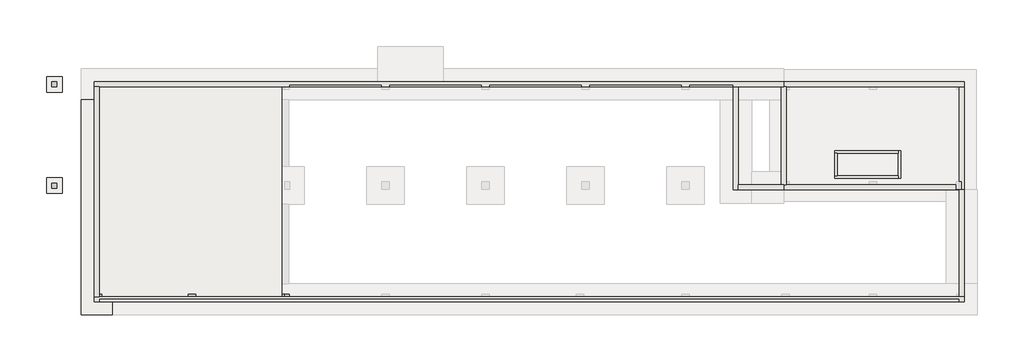
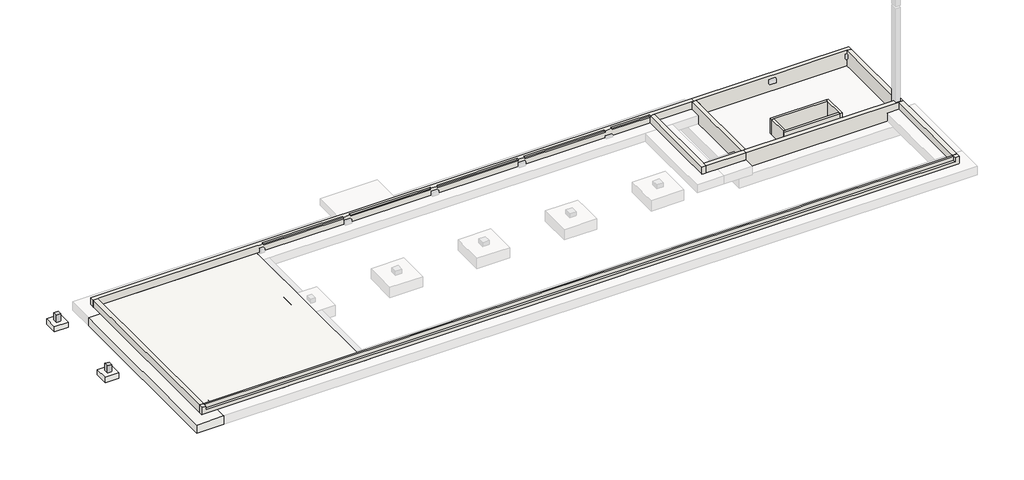
# Not in any storey, part 1 of 2: 14 walls, 5 columns, 3 slabs, 2 beams, 1 footing.
"""IFC4 building model written with IfcOpenShell, lengths in millimetres."""

import ifcopenshell
import ifcopenshell.guid

model = None  # the IFC model being written
_history = None  # IfcOwnerHistory: only IFC2X3 demands one
_inside = {}  # id of a spatial element -> (the spatial element, [elements in it])
_under = {}  # id of a project, library or spatial element -> (it, [spatial elements below it])
_declared = {}  # id of a project -> (the project, [libraries it declares])
_typed = {}  # id of a type object -> (the type object, [elements of that type])
_made_of = {}  # id of a material, layer set ... -> (it, [elements and type objects made of it])


def new_model(schema):
    """Start an empty IFC model of exactly this schema.

    Asked for "IFC4X3", IfcOpenShell would pick the latest addendum, in which some entities
    have other attributes; the version numbers below select the first issue.
    IFC2X3 requires an IfcOwnerHistory on every rooted entity: one is made here for all.
    """
    global model, _history
    if schema == "IFC4X3":
        model = ifcopenshell.file(schema_version=(4, 3, 0, 0))
    else:
        model = ifcopenshell.file(schema=schema)
    _inside.clear()
    _under.clear()
    _declared.clear()
    _typed.clear()
    _made_of.clear()
    _history = None
    if model.schema == "IFC2X3":
        org = make("IfcOrganization", Name="unknown")
        user = make(
            "IfcPersonAndOrganization",
            ThePerson=make("IfcPerson", FamilyName="unknown"),
            TheOrganization=org,
        )
        app = make(
            "IfcApplication",
            ApplicationDeveloper=org,
            Version="unknown",
            ApplicationFullName="unknown",
            ApplicationIdentifier="unknown",
        )
        _history = make(
            "IfcOwnerHistory",
            OwningUser=user,
            OwningApplication=app,
            ChangeAction="ADDED",
            CreationDate=0,
        )
    return model


def make(cls, **values):
    """One entity of the class cls with the attributes given. An attribute that is None is left unset."""
    return model.create_entity(
        cls, **{name: value for name, value in values.items() if value is not None}
    )


def rooted(cls, **values):
    """An entity with a GlobalId (a new one), such as an element, a storey or a relation."""
    return make(cls, GlobalId=ifcopenshell.guid.new(), OwnerHistory=_history, **values)


def si_unit(unit_type, name, prefix=None):
    """IfcSIUnit, for example si_unit("LENGTHUNIT", "METRE", prefix="MILLI")."""
    return make("IfcSIUnit", UnitType=unit_type, Prefix=prefix, Name=name)


def assignment(units):
    """IfcUnitAssignment: the units of a project."""
    return None if units is None else make("IfcUnitAssignment", Units=units)


def point(xyz):
    """IfcCartesianPoint."""
    return None if xyz is None else make("IfcCartesianPoint", Coordinates=xyz)


def direction(xyz):
    """IfcDirection."""
    return None if xyz is None else make("IfcDirection", DirectionRatios=xyz)


def frame(location, z_axis=None, x_axis=None):
    """IfcAxis2Placement3D, a coordinate frame: its origin and axes. An axis left out is left unset."""
    return make(
        "IfcAxis2Placement3D",
        Location=point(location),
        Axis=direction(z_axis),
        RefDirection=direction(x_axis),
    )


def origin():
    """The frame at (0, 0, 0) with its axes left unset."""
    return frame((0.0, 0.0, 0.0))


def place(relative_to, where):
    """IfcLocalPlacement: puts the frame where relative to a parent placement (None: the world)."""
    return make(
        "IfcLocalPlacement", PlacementRelTo=relative_to, RelativePlacement=where
    )


def context(
    kind, dimensions, precision=None, world=None, true_north=None, identifier=None
):
    """IfcGeometricRepresentationContext, for example the 3D "Model" context."""
    return make(
        "IfcGeometricRepresentationContext",
        ContextIdentifier=identifier,
        ContextType=kind,
        CoordinateSpaceDimension=dimensions,
        Precision=precision,
        WorldCoordinateSystem=world,
        TrueNorth=true_north,
    )


def project(units=None, contexts=None):
    """IfcProject with its units and contexts."""
    return rooted(
        "IfcProject",
        Name="project",
        RepresentationContexts=contexts,
        UnitsInContext=assignment(units),
    )


def spatial(cls, under=None, at=None, **own):
    """A site, building, storey or space (cls), placed at a placement, below another one or the project."""
    s = rooted(cls, ObjectPlacement=at, **own)
    if under is not None:
        _under.setdefault(under.id(), (under, []))[1].append(s)
    return s


def polyline(points):
    """IfcPolyline through the points."""
    return make("IfcPolyline", Points=[point(p) for p in points])


def outline(outer, holes=None, kind="AREA"):
    """IfcArbitraryClosedProfileDef: a profile drawn as a closed curve; with holes, ...WithVoids."""
    if holes is None:
        return make("IfcArbitraryClosedProfileDef", ProfileType=kind, OuterCurve=outer)
    return make(
        "IfcArbitraryProfileDefWithVoids",
        ProfileType=kind,
        OuterCurve=outer,
        InnerCurves=holes,
    )


def extrude(swept, where, along, depth):
    """IfcExtrudedAreaSolid: the profile swept, set in the frame where, extruded along a direction by depth."""
    return make(
        "IfcExtrudedAreaSolid",
        SweptArea=swept,
        Position=where,
        ExtrudedDirection=direction(along),
        Depth=depth,
    )


def faces_of(points, faces, orient=None, outer=None):
    """IfcFace entities. A face is a list of loops; a loop is a list of indices into points, from 0.

    orient and outer hold one flag for each loop. By default every Orientation is true, the
    first loop of a face is its IfcFaceOuterBound and the others are IfcFaceBound.
    """
    made = []
    for i, loops in enumerate(faces):
        bounds = []
        for j, loop in enumerate(loops):
            is_outer = j == 0 if outer is None else outer[i][j]
            bounds.append(
                make(
                    "IfcFaceOuterBound" if is_outer else "IfcFaceBound",
                    Bound=make("IfcPolyLoop", Polygon=[points[k] for k in loop]),
                    Orientation=True if orient is None else orient[i][j],
                )
            )
        made.append(make("IfcFace", Bounds=bounds))
    return made


def faceted_brep(points, faces, orient=None, outer=None, voids=None):
    """IfcFacetedBrep: a solid bounded by flat faces; with voids (closed shells), ...WithVoids."""
    shared = [point(p) for p in points]
    hull = make("IfcClosedShell", CfsFaces=faces_of(shared, faces, orient, outer))
    if voids is None:
        return make("IfcFacetedBrep", Outer=hull)
    return make(
        "IfcFacetedBrepWithVoids",
        Outer=hull,
        Voids=[
            make(cls, CfsFaces=faces_of(shared, fs, o, b)) for cls, fs, o, b in voids
        ],
    )


def shape(context_of_items, identifier, shape_type, items):
    """IfcShapeRepresentation: the items that make up one representation, for example the "Body"."""
    return make(
        "IfcShapeRepresentation",
        ContextOfItems=context_of_items,
        RepresentationIdentifier=identifier,
        RepresentationType=shape_type,
        Items=items,
    )


def source(mapping_origin, context_of_items, identifier, shape_type, items):
    """IfcRepresentationMap: a shape defined once, which mapped items show again and again."""
    return make(
        "IfcRepresentationMap",
        MappingOrigin=mapping_origin,
        MappedRepresentation=shape(context_of_items, identifier, shape_type, items),
    )


def transform(
    local_origin,
    x_axis=None,
    y_axis=None,
    z_axis=None,
    scale=None,
    scale2=None,
    scale3=None,
    uniform=True,
):
    """IfcCartesianTransformationOperator3D, or its non-uniform kind. x_axis, y_axis, z_axis: its Axis1, 2, 3."""
    if uniform:
        return make(
            "IfcCartesianTransformationOperator3D",
            Axis1=direction(x_axis),
            Axis2=direction(y_axis),
            LocalOrigin=point(local_origin),
            Scale=scale,
            Axis3=direction(z_axis),
        )
    return make(
        "IfcCartesianTransformationOperator3DnonUniform",
        Axis1=direction(x_axis),
        Axis2=direction(y_axis),
        LocalOrigin=point(local_origin),
        Scale=scale,
        Axis3=direction(z_axis),
        Scale2=scale2,
        Scale3=scale3,
    )


def mapped(mapping_source, mapping_target):
    """IfcMappedItem: shows the shape of a source again, moved by a transform."""
    return make(
        "IfcMappedItem", MappingSource=mapping_source, MappingTarget=mapping_target
    )


def made_of(thing, what):
    """Note that an element or type object is made of a material, layer set ...; save() writes the relation."""
    if what is not None:
        _made_of.setdefault(what.id(), (what, []))[1].append(thing)
    return thing


def element(
    cls,
    number,
    at=None,
    inside=None,
    cuts=None,
    type_object=None,
    material=None,
    context=None,
    identifier="Body",
    shape_type=None,
    held_by="IfcProductDefinitionShape",
    body=None,
    shapes=None,
    **own,
):
    """One element of the class cls, such as IfcWall. Its Tag is "e" and its number.

    at: its placement. inside: the storey or other place that contains it. cuts: it is an
    opening in that element (IfcRelVoidsElement). A single representation is given by context,
    identifier, shape_type and body (its items); several are given by shapes. held_by: the class
    of the entity that holds the representations. save() writes the other relations.
    """
    e = rooted(cls, Tag="e%d" % number, ObjectPlacement=at, **own)
    if body is not None:
        shapes = [shape(context, identifier, shape_type, body)]
    if shapes is not None:
        e.Representation = make(held_by, Representations=shapes)
    if inside is not None:
        _inside.setdefault(inside.id(), (inside, []))[1].append(e)
    if cuts is not None:
        rooted(
            "IfcRelVoidsElement", RelatingBuildingElement=cuts, RelatedOpeningElement=e
        )
    if type_object is not None:
        _typed.setdefault(type_object.id(), (type_object, []))[1].append(e)
    return made_of(e, material)


def aggregate(whole, parts):
    """IfcRelAggregates: a whole, such as a stair, and the parts it consists of."""
    return rooted("IfcRelAggregates", RelatingObject=whole, RelatedObjects=parts)


def save(model, path):
    """Write the relations noted so far, then the file.

    IfcRelAggregates (storeys below a building ...), IfcRelContainedInSpatialStructure (elements
    in a storey), IfcRelDefinesByType, IfcRelAssociatesMaterial and IfcRelDeclares: one each for
    every whole, place, type object, material and project.
    """
    for whole, parts in _under.values():
        aggregate(whole, parts)
    for where, things in _inside.values():
        rooted(
            "IfcRelContainedInSpatialStructure",
            RelatedElements=things,
            RelatingStructure=where,
        )
    for kind, things in _typed.values():
        rooted("IfcRelDefinesByType", RelatedObjects=things, RelatingType=kind)
    for what, things in _made_of.values():
        rooted("IfcRelAssociatesMaterial", RelatedObjects=things, RelatingMaterial=what)
    for by, libraries in _declared.values():
        rooted("IfcRelDeclares", RelatingContext=by, RelatedDefinitions=libraries)
    model.write(path)


def foundation_rectangular_non_pile_17b72d6a(model_context):
    return source(origin(), model_context, "Body", "SweptSolid", [
        extrude(outline(polyline([(625.0, 625.0), (625.0, -625.0), (-625.0, -625.0), (-625.0, 625.0), (625.0, 625.0)])), frame((0.0, 0.0, -500.0), z_axis=(0.0, 0.0, 1.0), x_axis=(1.0, 0.0, 0.0)), (0.0, 0.0, 1.0), 500.0),
    ])


model = new_model("IFC4")

# Units and contexts
model_context = context("Model", 3, world=origin())
ifc_project = project(units=[si_unit("LENGTHUNIT", "METRE", prefix="MILLI")], contexts=[model_context])

# Site, building
site = spatial("IfcSite", under=ifc_project)
building = spatial("IfcBuilding", under=site)

# Beams
placement = place(None, origin())
element("IfcBeam", 1, ObjectType="RC Beam_Rectangular : H_SB_AR_S16_FG_B500xH700_FB1", at=placement, inside=building, context=model_context, shape_type="SweptSolid", body=[
    extrude(outline(polyline([(3500.0, 9199.5208589), (4000.0, 9199.5208589), (4000.0, 1649.5208589), (3500.0, 1649.5208589), (3500.0, 9199.5208589)])), frame((0.0, 0.0, -1250.0381366), z_axis=(0.0, 0.0, 1.0), x_axis=(1.0, 0.0, 0.0)), (0.0, 0.0, 1.0), 550.0),
])
element("IfcBeam", 2, ObjectType="RC Beam_Rectangular : H_SB_AR_S16_FG_B500xH700_FG1", at=placement, inside=building, context=model_context, shape_type="SweptSolid", body=[
    extrude(outline(polyline([(7750.0, 1649.5208589), (7250.0, 1649.5208589), (7250.0, 7999.5208589), (7750.0, 7999.5208589), (7750.0, 1649.5208589)])), frame((0.0, 0.0, -1250.0381366), z_axis=(0.0, 0.0, 1.0), x_axis=(1.0, 0.0, 0.0)), (0.0, 0.0, 1.0), 550.0),
])

# Columns
element("IfcColumn", 3, ObjectType="RC_Column_Rectangular : H_SC_AR_S15_UG_W600xL600_C2", at=placement, inside=building, context=model_context, shape_type="Brep", body=[
    faceted_brep([(15300.0, 799.5208589, -850.0381366), (15300.0, 199.5208589, -850.0381366), (14700.0, 199.5208589, -850.0381366), (14700.0, 799.5208589, -850.0381366), (15300.0, 799.5208589, -150.0381366), (15300.0, 599.5208589, -150.0381366), (15300.0, 599.5208589, -550.0381366), (15300.0, 199.5208589, -550.0381366), (14700.0, 199.5208589, -550.0381366), (14700.0, 599.5208589, -550.0381366), (14700.0, 799.5208589, -550.0381366), (14950.0, 799.5208589, -550.0381366), (14950.0, 799.5208589, -150.0381366), (14950.0, 599.5208589, -150.0381366), (14950.0, 599.5208589, -550.0381366)], [[[0, 1, 2, 3]], [[1, 0, 4, 5, 6, 7]], [[2, 1, 7, 8]], [[3, 2, 8, 9, 10]], [[0, 3, 10, 11, 12, 4]], [[5, 4, 12, 13]], [[6, 5, 13, 14]], [[7, 6, 14, 11, 10, 9, 8]], [[11, 14, 13, 12]]]),
])
element("IfcColumn", 4, ObjectType="RC_Column_Rectangular : H_SC_AR_S15_UG_W600xL600_C2", at=placement, inside=building, context=model_context, shape_type="Brep", body=[
    faceted_brep([(7800.0, 799.5208589, -850.0381366), (7800.0, 199.5208589, -850.0381366), (7200.0, 199.5208589, -850.0381366), (7200.0, 799.5208589, -850.0381366), (7800.0, 599.5208589, -150.0381366), (7800.0, 599.5208589, -550.0381366), (7800.0, 799.5208589, -550.0381366), (7800.0, 799.5208589, -150.0381366), (7800.0, 199.5208589, -550.0381366), (7200.0, 199.5208589, -550.0381366), (7200.0, 599.5208589, -550.0381366), (7200.0, 599.5208589, -150.0381366), (7200.0, 799.5208589, -150.0381366), (7200.0, 799.5208589, -550.0381366), (7200.0, 599.5208589, -700.0381366), (7800.0, 599.5208589, -700.0381366), (7800.0, 799.5208589, -700.0381366), (7200.0, 799.5208589, -700.0381366)], [[[0, 1, 2, 3]], [[4, 5, 6, 7]], [[2, 1, 8, 9]], [[10, 11, 12, 13]], [[12, 7, 6, 13]], [[7, 12, 11, 4]], [[10, 5, 4, 11]], [[5, 10, 9, 8]], [[14, 15, 16, 17]], [[5, 10, 13, 6]], [[10, 5, 15, 14]], [[1, 0, 16, 15, 5, 8]], [[3, 2, 9, 10, 14, 17]], [[0, 3, 17, 16]]]),
])
element("IfcColumn", 5, ObjectType="RC_Column_Rectangular : H_SC_AR_S15_UG_W600xL600_C2", at=placement, inside=building, context=model_context, shape_type="Brep", body=[
    faceted_brep([(300.0, 799.5208589, -850.0381366), (300.0, 199.5208589, -850.0381366), (-300.0, 199.5208589, -850.0381366), (-300.0, 799.5208589, -850.0381366), (300.0, 599.5208589, -150.0381366), (300.0, 599.5208589, -550.0381366), (300.0, 799.5208589, -550.0381366), (300.0, 799.5208589, -150.0381366), (300.0, 199.5208589, -550.0381366), (-300.0, 199.5208589, -550.0381366), (-300.0, 599.5208589, -550.0381366), (-300.0, 799.5208589, -550.0381366), (100.0, 799.5208589, -550.0381366), (100.0, 799.5208589, -150.0381366), (100.0, 599.5208589, -150.0381366), (100.0, 599.5208589, -550.0381366), (100.0, 799.5208589, -700.0381366), (100.0, 599.5208589, -700.0381366), (300.0, 599.5208589, -700.0381366), (300.0, 799.5208589, -700.0381366), (100.0, 599.5208589, -550.0381366)], [[[0, 1, 2, 3]], [[4, 5, 6, 7]], [[2, 1, 8, 9]], [[3, 2, 9, 10, 11]], [[12, 13, 7, 6]], [[4, 7, 13, 14]], [[5, 4, 14, 15]], [[8, 5, 15, 12, 11, 10, 9]], [[12, 15, 14, 13]], [[16, 17, 18, 19]], [[5, 20, 12, 6]], [[17, 20, 5, 18]], [[20, 17, 16, 12]], [[1, 0, 19, 18, 5, 8]], [[0, 3, 11, 12, 16, 19]]]),
])
element("IfcColumn", 6, ObjectType="RC_Column_Rectangular : H_SC_AR_S15_UG_W400xL400_C3", at=placement, inside=building, context=model_context, shape_type="SweptSolid", body=[
    extrude(outline(polyline([(-3300.0, 9699.5208589), (-3300.0, 9299.5208589), (-3700.0, 9299.5208589), (-3700.0, 9699.5208589), (-3300.0, 9699.5208589)])), frame((0.0, 0.0, -850.0381366), z_axis=(0.0, 0.0, 1.0), x_axis=(1.0, 0.0, 0.0)), (0.0, 0.0, 1.0), 700.0),
])
element("IfcColumn", 7, ObjectType="RC_Column_Rectangular : H_SC_AR_S15_UG_W400xL400_C3", at=placement, inside=building, context=model_context, shape_type="Brep", body=[
    faceted_brep([(-3300.0, 17799.5208589, -850.0381366), (-3300.0, 17399.5208589, -850.0381366), (-3700.0, 17399.5208589, -850.0381366), (-3700.0, 17799.5208589, -850.0381366), (-3300.0, 17799.5208589, -150.0381366), (-3300.0, 17399.5208589, -150.0381366), (-3300.0, 17399.5208589, -550.0381366), (-3300.0, 17799.5208589, -550.0381366), (-3700.0, 17399.5208589, -150.0381366), (-3700.0, 17799.5208589, -150.0381366)], [[[0, 1, 2, 3]], [[4, 5, 6, 1, 0, 7]], [[5, 8, 2, 1, 6]], [[8, 9, 3, 2]], [[9, 4, 7, 0, 3]], [[4, 9, 8, 5]]]),
])

# Footing
element("IfcFooting", 8, ObjectType="H_SF_AR_B01_Wall FDN_T800", at=placement, inside=building, context=model_context, shape_type="Brep", body=[
    faceted_brep([(-1350.0, -850.4791411, -550.0381366), (1150.0, -850.4791411, -550.0381366), (1150.0, 1649.5208589, -550.0381366), (1150.0, 16349.5208589, -550.0381366), (-1350.0, 16349.5208589, -550.0381366), (-1350.0, -850.4791411, -1350.0381366), (-1350.0, 16349.5208589, -1350.0381366), (1150.0, -850.4791411, -1350.0381366), (1150.0, 16349.5208589, -1350.0381366), (1150.0, 9799.5208589, -1350.0381366), (1150.0, 9199.5208589, -1350.0381366), (1150.0, 1649.5208589, -1350.0381366)], [[[0, 1, 2, 3, 4]], [[5, 0, 4, 6]], [[7, 5, 6, 8, 9, 10, 11]], [[1, 7, 11, 10, 9, 8, 3, 2]], [[1, 0, 5, 7]], [[4, 3, 8, 6]]]),
])

# Slabs
element("IfcSlab", 9, ObjectType="H_FL_AR_S17_RC Slab T150_B1S1", at=placement, inside=building, context=model_context, shape_type="Brep", body=[
    faceted_brep([(14700.0, 17399.5208589, -700.0381366), (14700.0, 599.5208589, -700.0381366), (7800.0, 599.5208589, -700.0381366), (7200.0, 599.5208589, -700.0381366), (300.0, 599.5208589, -700.0381366), (100.0, 599.5208589, -700.0381366), (100.0, 799.5208589, -700.0381366), (100.0, 17199.5208589, -700.0381366), (100.0, 17399.5208589, -700.0381366), (300.0, 17399.5208589, -700.0381366), (7200.0, 17399.5208589, -700.0381366), (7800.0, 17399.5208589, -700.0381366), (14700.0, 17399.5208589, -550.0381366), (7800.0, 17399.5208589, -550.0381366), (7200.0, 17399.5208589, -550.0381366), (300.0, 17399.5208589, -550.0381366), (100.0, 17399.5208589, -550.0381366), (100.0, 17199.5208589, -550.0381366), (100.0, 799.5208589, -550.0381366), (100.0, 599.5208589, -550.0381366), (300.0, 599.5208589, -550.0381366), (7200.0, 599.5208589, -550.0381366), (7800.0, 599.5208589, -550.0381366), (14700.0, 599.5208589, -550.0381366), (14700.0, 799.5208589, -550.0381366), (14700.0, 17199.5208589, -550.0381366)], [[[0, 1, 2, 3, 4, 5, 6, 7, 8, 9, 10, 11]], [[12, 13, 14, 15, 16, 17, 18, 19, 20, 21, 22, 23, 24, 25]], [[1, 0, 12, 25, 24, 23]], [[5, 4, 3, 2, 1, 23, 22, 21, 20, 19]], [[8, 7, 6, 5, 19, 18, 17, 16]], [[0, 11, 10, 9, 8, 16, 15, 14, 13, 12]]]),
])
element("IfcSlab", 10, ObjectType="Foundation Rectangular (Non-Pile) : H_SF_AR_S18_W1250xL1250xT500_Bitumen_F2", at=placement, inside=building, context=model_context, shape_type="SweptSolid", body=[
    extrude(outline(polyline([(-2875.0, 18224.5208589), (-2875.0, 16974.5208589), (-4125.0, 16974.5208589), (-4125.0, 18224.5208589), (-2875.0, 18224.5208589)])), frame((0.0, 0.0, -1350.0381366), z_axis=(0.0, 0.0, 1.0), x_axis=(1.0, 0.0, 0.0)), (0.0, 0.0, 1.0), 500.0),
])
foundation_rectangular_non_pile_shape = foundation_rectangular_non_pile_17b72d6a(model_context)
element("IfcSlab", 11, ObjectType="Foundation Rectangular (Non-Pile) : H_SF_AR_S18_W1250xL1250xT500_Bitumen_F2", at=placement, inside=building, context=model_context, shape_type="MappedRepresentation", body=[
    mapped(foundation_rectangular_non_pile_shape, transform((-3500.0, 9499.5208589, -850.0381366), x_axis=(1.0, 0.0, 0.0), y_axis=(0.0, 1.0, 0.0), z_axis=(0.0, 0.0, 1.0))),
])

# Walls
element("IfcWall", 12, ObjectType="H_WA_AR_B02_Ext Wall_RC T400_UG_Bitumen 2", at=placement, inside=building, context=model_context, shape_type="Brep", body=[
    faceted_brep([(-300.0, 17399.5208589, -550.0381366), (100.0, 17399.5208589, -550.0381366), (300.0, 17399.5208589, -550.0381366), (7200.0, 17399.5208589, -550.0381366), (7800.0, 17399.5208589, -550.0381366), (14700.0, 17399.5208589, -550.0381366), (14950.0, 17399.5208589, -550.0381366), (15300.0, 17399.5208589, -550.0381366), (22700.0, 17399.5208589, -550.0381366), (23300.0, 17399.5208589, -550.0381366), (30700.0, 17399.5208589, -550.0381366), (31300.0, 17399.5208589, -550.0381366), (38700.0, 17399.5208589, -550.0381366), (39300.0, 17399.5208589, -550.0381366), (46700.0, 17399.5208589, -550.0381366), (47300.0, 17399.5208589, -550.0381366), (50825.0, 17399.5208589, -550.0381366), (51225.0, 17399.5208589, -550.0381366), (54650.0, 17399.5208589, -550.0381366), (54850.0, 17399.5208589, -550.0381366), (54850.0, 17399.5208589, 149.9618634), (54650.0, 17399.5208589, 149.9618634), (51225.0, 17399.5208589, 149.9618634), (50825.0, 17399.5208589, 149.9618634), (50825.0, 17399.5208589, -0.0381366), (47300.0, 17399.5208589, -0.0381366), (47300.0, 17399.5208589, 149.9618634), (46700.0, 17399.5208589, 149.9618634), (46700.0, 17399.5208589, -0.0381366), (39300.0, 17399.5208589, -0.0381366), (39300.0, 17399.5208589, 149.9618634), (38700.0, 17399.5208589, 149.9618634), (38700.0, 17399.5208589, -0.0381366), (31300.0, 17399.5208589, -0.0381366), (31300.0, 17399.5208589, 149.9618634), (30700.0, 17399.5208589, 149.9618634), (30700.0, 17399.5208589, -0.0381366), (23300.0, 17399.5208589, -0.0381366), (23300.0, 17399.5208589, 149.9618634), (22700.0, 17399.5208589, 149.9618634), (22700.0, 17399.5208589, -0.0381366), (15300.0, 17399.5208589, -0.0381366), (15300.0, 17399.5208589, 149.9618634), (14950.0, 17399.5208589, 149.9618634), (14700.0, 17399.5208589, 149.9618634), (7800.0, 17399.5208589, 149.9618634), (7200.0, 17399.5208589, 149.9618634), (300.0, 17399.5208589, 149.9618634), (100.0, 17399.5208589, 149.9618634), (-300.0, 17399.5208589, 149.9618634), (-300.0, 17399.5208589, -20.0381366), (54850.0, 17799.5208589, -550.0381366), (54650.0, 17799.5208589, -550.0381366), (47300.0, 17799.5208589, -550.0381366), (46700.0, 17799.5208589, -550.0381366), (39300.0, 17799.5208589, -550.0381366), (38700.0, 17799.5208589, -550.0381366), (31300.0, 17799.5208589, -550.0381366), (30700.0, 17799.5208589, -550.0381366), (23300.0, 17799.5208589, -550.0381366), (22700.0, 17799.5208589, -550.0381366), (15300.0, 17799.5208589, -550.0381366), (14700.0, 17799.5208589, -550.0381366), (7800.0, 17799.5208589, -550.0381366), (7200.0, 17799.5208589, -550.0381366), (300.0, 17799.5208589, -550.0381366), (-300.0, 17799.5208589, -550.0381366), (-300.0, 17799.5208589, -20.0381366), (-300.0, 17799.5208589, 149.9618634), (18450.0, 17799.5208589, 149.9618634), (19550.0, 17799.5208589, 149.9618634), (24050.0, 17799.5208589, 149.9618634), (26150.0, 17799.5208589, 149.9618634), (54850.0, 17799.5208589, 149.9618634), (-300.0, 17549.5208589, 149.9618634), (15300.0, 17549.5208589, 149.9618634), (22700.0, 17549.5208589, 149.9618634), (23300.0, 17549.5208589, 149.9618634), (30700.0, 17549.5208589, 149.9618634), (31300.0, 17549.5208589, 149.9618634), (38700.0, 17549.5208589, 149.9618634), (39300.0, 17549.5208589, 149.9618634), (46700.0, 17549.5208589, 149.9618634), (47300.0, 17549.5208589, 149.9618634), (50825.0, 17549.5208589, 149.9618634), (22700.0, 17549.5208589, -0.0381366), (15300.0, 17549.5208589, -0.0381366), (30700.0, 17549.5208589, -0.0381366), (23300.0, 17549.5208589, -0.0381366), (38700.0, 17549.5208589, -0.0381366), (31300.0, 17549.5208589, -0.0381366), (46700.0, 17549.5208589, -0.0381366), (39300.0, 17549.5208589, -0.0381366), (50825.0, 17549.5208589, -0.0381366), (47300.0, 17549.5208589, -0.0381366)], [[[0, 1, 2, 3, 4, 5, 6, 7, 8, 9, 10, 11, 12, 13, 14, 15, 16, 17, 18, 19, 20, 21, 22, 23, 24, 25, 26, 27, 28, 29, 30, 31, 32, 33, 34, 35, 36, 37, 38, 39, 40, 41, 42, 43, 44, 45, 46, 47, 48, 49, 50]], [[51, 52, 53, 54, 55, 56, 57, 58, 59, 60, 61, 62, 63, 64, 65, 66, 67, 68, 69, 70, 71, 72, 73]], [[19, 18, 17, 16, 15, 14, 13, 12, 11, 10, 9, 8, 7, 6, 5, 4, 3, 2, 1, 0, 66, 65, 64, 63, 62, 61, 60, 59, 58, 57, 56, 55, 54, 53, 52, 51]], [[20, 19, 51, 73]], [[73, 72, 71, 70, 69, 68, 74, 49, 48, 47, 46, 45, 44, 43, 42, 75, 76, 39, 38, 77, 78, 35, 34, 79, 80, 31, 30, 81, 82, 27, 26, 83, 84, 23, 22, 21, 20]], [[49, 74, 68, 67, 66, 0, 50]], [[85, 86, 41, 40]], [[87, 88, 37, 36]], [[89, 90, 33, 32]], [[91, 92, 29, 28]], [[93, 94, 25, 24]], [[86, 75, 42, 41]], [[86, 85, 76, 75]], [[76, 85, 40, 39]], [[88, 77, 38, 37]], [[88, 87, 78, 77]], [[78, 87, 36, 35]], [[90, 79, 34, 33]], [[90, 89, 80, 79]], [[80, 89, 32, 31]], [[92, 81, 30, 29]], [[92, 91, 82, 81]], [[82, 91, 28, 27]], [[94, 83, 26, 25]], [[94, 93, 84, 83]], [[84, 93, 24, 23]]]),
])
element("IfcWall", 13, ObjectType="H_WA_AR_B02_Ext Wall_RC T400_UG_Bitumen 2", at=placement, inside=building, context=model_context, shape_type="Brep", body=[
    faceted_brep([(69300.0, 599.5208589, -550.0381366), (68900.0, 599.5208589, -550.0381366), (68700.0, 599.5208589, -550.0381366), (62300.0, 599.5208589, -550.0381366), (61700.0, 599.5208589, -550.0381366), (55300.0, 599.5208589, -550.0381366), (54700.0, 599.5208589, -550.0381366), (47300.0, 599.5208589, -550.0381366), (46700.0, 599.5208589, -550.0381366), (39240.1112654, 599.5208589, -550.0381366), (38850.0, 599.5208589, -550.0381366), (38250.0, 599.5208589, -550.0381366), (31300.0, 599.5208589, -550.0381366), (30700.0, 599.5208589, -550.0381366), (23300.0, 599.5208589, -550.0381366), (22700.0, 599.5208589, -550.0381366), (15300.0, 599.5208589, -550.0381366), (14950.0, 599.5208589, -550.0381366), (14700.0, 599.5208589, -550.0381366), (7800.0, 599.5208589, -550.0381366), (7200.0, 599.5208589, -550.0381366), (300.0, 599.5208589, -550.0381366), (100.0, 599.5208589, -550.0381366), (-300.0, 599.5208589, -550.0381366), (-300.0, 599.5208589, 149.9618634), (100.0, 599.5208589, 149.9618634), (300.0, 599.5208589, 149.9618634), (7200.0, 599.5208589, 149.9618634), (7800.0, 599.5208589, 149.9618634), (14700.0, 599.5208589, 149.9618634), (14950.0, 599.5208589, 149.9618634), (15300.0, 599.5208589, 149.9618634), (22700.0, 599.5208589, 149.9618634), (23300.0, 599.5208589, 149.9618634), (30700.0, 599.5208589, 149.9618634), (31300.0, 599.5208589, 149.9618634), (38700.0, 599.5208589, 149.9618634), (39300.0, 599.5208589, 149.9618634), (46700.0, 599.5208589, 149.9618634), (47300.0, 599.5208589, 149.9618634), (54700.0, 599.5208589, 149.9618634), (55300.0, 599.5208589, 149.9618634), (61700.0, 599.5208589, 149.9618634), (62300.0, 599.5208589, 149.9618634), (68700.0, 599.5208589, 149.9618634), (68900.0, 599.5208589, 149.9618634), (69300.0, 599.5208589, 149.9618634), (-300.0, 199.5208589, -550.0381366), (300.0, 199.5208589, -550.0381366), (7200.0, 199.5208589, -550.0381366), (7800.0, 199.5208589, -550.0381366), (14700.0, 199.5208589, -550.0381366), (15300.0, 199.5208589, -550.0381366), (22700.0, 199.5208589, -550.0381366), (23300.0, 199.5208589, -550.0381366), (30700.0, 199.5208589, -550.0381366), (31300.0, 199.5208589, -550.0381366), (38250.0, 199.5208589, -550.0381366), (38850.0, 199.5208589, -550.0381366), (46700.0, 199.5208589, -550.0381366), (47300.0, 199.5208589, -550.0381366), (54700.0, 199.5208589, -550.0381366), (55300.0, 199.5208589, -550.0381366), (61700.0, 199.5208589, -550.0381366), (62300.0, 199.5208589, -550.0381366), (68700.0, 199.5208589, -550.0381366), (69300.0, 199.5208589, -550.0381366), (69300.0, 199.5208589, 149.9618634), (68900.0, 199.5208589, 149.9618634), (68900.0, 199.5208589, -231.142699), (100.0, 199.5208589, -231.142699), (100.0, 199.5208589, 149.9618634), (-50.0, 199.5208589, 149.9618634), (-300.0, 199.5208589, 149.9618634), (100.0, 449.5208589, 149.9618634), (300.0, 449.5208589, 149.9618634), (7200.0, 449.5208589, 149.9618634), (7800.0, 449.5208589, 149.9618634), (14700.0, 449.5208589, 149.9618634), (15300.0, 449.5208589, 149.9618634), (22700.0, 449.5208589, 149.9618634), (23300.0, 449.5208589, 149.9618634), (30700.0, 449.5208589, 149.9618634), (31300.0, 449.5208589, 149.9618634), (38700.0, 449.5208589, 149.9618634), (39300.0, 449.5208589, 149.9618634), (46700.0, 449.5208589, 149.9618634), (47300.0, 449.5208589, 149.9618634), (53150.0, 449.5208589, 149.9618634), (54150.0, 449.5208589, 149.9618634), (54700.0, 449.5208589, 149.9618634), (55300.0, 449.5208589, 149.9618634), (61700.0, 449.5208589, 149.9618634), (62300.0, 449.5208589, 149.9618634), (68700.0, 449.5208589, 149.9618634), (68900.0, 449.5208589, 149.9618634), (69300.0, 449.5208589, 149.9618634), (100.0, 449.5208589, -231.142699), (68900.0, 449.5208589, -231.142699)], [[[0, 1, 2, 3, 4, 5, 6, 7, 8, 9, 10, 11, 12, 13, 14, 15, 16, 17, 18, 19, 20, 21, 22, 23, 24, 25, 26, 27, 28, 29, 30, 31, 32, 33, 34, 35, 36, 37, 38, 39, 40, 41, 42, 43, 44, 45, 46]], [[47, 48, 49, 50, 51, 52, 53, 54, 55, 56, 57, 58, 59, 60, 61, 62, 63, 64, 65, 66, 67, 68, 69, 70, 71, 72, 73]], [[23, 22, 21, 20, 19, 18, 17, 16, 15, 14, 13, 12, 11, 10, 9, 8, 7, 6, 5, 4, 3, 2, 1, 0, 66, 65, 64, 63, 62, 61, 60, 59, 58, 57, 56, 55, 54, 53, 52, 51, 50, 49, 48, 47]], [[46, 45, 44, 43, 42, 41, 40, 39, 38, 37, 36, 35, 34, 33, 32, 31, 30, 29, 28, 27, 26, 25, 24, 73, 72, 71, 74, 75, 76, 77, 78, 79, 80, 81, 82, 83, 84, 85, 86, 87, 88, 89, 90, 91, 92, 93, 94, 95, 68, 67, 96]], [[23, 47, 73, 24]], [[66, 0, 46, 96, 67]], [[97, 98, 95, 94, 93, 92, 91, 90, 89, 88, 87, 86, 85, 84, 83, 82, 81, 80, 79, 78, 77, 76, 75, 74]], [[98, 97, 70, 69]], [[97, 74, 71, 70]], [[95, 98, 69, 68]]]),
])
element("IfcWall", 14, ObjectType="H_WA_AR_B02_Ext Wall_RC T400_UG_Bitumen 2", at=placement, inside=building, context=model_context, shape_type="Brep", body=[
    faceted_brep([(100.0, 599.5208589, 149.9618634), (100.0, 599.5208589, -150.0381366), (100.0, 599.5208589, -550.0381366), (100.0, 799.5208589, -550.0381366), (100.0, 17199.5208589, -550.0381366), (100.0, 17399.5208589, -550.0381366), (100.0, 17399.5208589, -150.0381366), (100.0, 17399.5208589, 149.9618634), (100.0, 17199.5208589, 149.9618634), (100.0, 9849.5208589, 149.9618634), (100.0, 9149.5208589, 149.9618634), (100.0, 799.5208589, 149.9618634), (-300.0, 599.5208589, -550.0381366), (-300.0, 599.5208589, 149.9618634), (-300.0, 17399.5208589, 149.9618634), (-300.0, 17399.5208589, -550.0381366), (-300.0, 17199.5208589, -550.0381366), (-300.0, 9699.5208589, -550.0381366), (-300.0, 9299.5208589, -550.0381366), (-300.0, 799.5208589, -550.0381366)], [[[0, 1, 2, 3, 4, 5, 6, 7, 8, 9, 10, 11]], [[12, 13, 14, 15, 16, 17, 18, 19]], [[5, 4, 3, 2, 12, 19, 18, 17, 16, 15]], [[0, 11, 10, 9, 8, 7, 14, 13]], [[5, 15, 14, 7, 6]], [[0, 13, 12, 2, 1]]]),
])
element("IfcWall", 15, ObjectType="H_WA_AR_B02_Ext Wall_RC T400_UG_Bitumen 2", at=placement, inside=building, context=model_context, shape_type="Brep", body=[
    faceted_brep([(68900.0, 9149.5208589, -550.0381366), (68900.0, 799.5208589, -550.0381366), (68900.0, 599.5208589, -550.0381366), (68900.0, 599.5208589, -150.0381366), (68900.0, 599.5208589, 149.9618634), (68900.0, 799.5208589, 149.9618634), (68900.0, 9149.5208589, 149.9618634), (69300.0, 9149.5208589, -550.0381366), (69300.0, 9149.5208589, 149.9618634), (69300.0, 7249.5208589, 149.9618634), (69300.0, 4149.5208589, 149.9618634), (69300.0, 599.5208589, 149.9618634), (69300.0, 599.5208589, -550.0381366), (69300.0, 799.5208589, -550.0381366)], [[[0, 1, 2, 3, 4, 5, 6]], [[7, 8, 9, 10, 11, 12, 13]], [[2, 1, 0, 7, 13, 12]], [[6, 5, 4, 11, 10, 9, 8]], [[0, 6, 8, 7]], [[2, 12, 11, 4, 3]]]),
])
element("IfcWall", 16, ObjectType="H_WA_AR_B02_Ext Wall_RC T400_UG_Bitumen 2", at=placement, inside=building, context=model_context, shape_type="Brep", body=[
    faceted_brep([(50825.0, 17399.5208589, -550.0381366), (50825.0, 9799.5208589, -550.0381366), (50825.0, 9149.5208589, -550.0381366), (50825.0, 9149.5208589, -0.0381366), (50825.0, 9149.5208589, 149.9618634), (50825.0, 9399.5208589, 149.9618634), (50825.0, 17399.5208589, 149.9618634), (51225.0, 17399.5208589, -550.0381366), (51225.0, 17399.5208589, 149.9618634), (51225.0, 9549.5208589, 149.9618634), (51225.0, 9399.5208589, 149.9618634), (51225.0, 9149.5208589, 149.9618634), (51225.0, 9149.5208589, -150.0381366), (51225.0, 9149.5208589, -550.0381366), (51225.0, 9549.5208589, -550.0381366), (51225.0, 9799.5208589, -550.0381366), (51175.0, 9149.5208589, -550.0381366)], [[[0, 1, 2, 3, 4, 5, 6]], [[7, 8, 9, 10, 11, 12, 13, 14, 15]], [[2, 1, 0, 7, 15, 14, 13, 16]], [[6, 5, 4, 11, 10, 9, 8]], [[0, 6, 8, 7]], [[2, 16, 13, 12, 11, 4, 3]]]),
])
element("IfcWall", 17, ObjectType="H_WA_AR_B02_Ext Wall_RC T400_UG_Bitumen 2", at=placement, inside=building, context=model_context, shape_type="Brep", body=[
    faceted_brep([(51225.0, 9149.5208589, 149.9618634), (51225.0, 9149.5208589, -550.0381366), (54650.0, 9149.5208589, -550.0381366), (54700.0, 9149.5208589, -550.0381366), (54850.0, 9149.5208589, -550.0381366), (54850.0, 9149.5208589, 149.9618634), (51225.0, 9549.5208589, -550.0381366), (51225.0, 9549.5208589, -50.0381366), (51225.0, 9549.5208589, 149.9618634), (54650.0, 9549.5208589, 149.9618634), (54850.0, 9549.5208589, 149.9618634), (54850.0, 9549.5208589, -550.0381366), (54650.0, 9549.5208589, -550.0381366)], [[[0, 1, 2, 3, 4, 5]], [[6, 7, 8, 9, 10, 11, 12]], [[4, 3, 2, 1, 6, 12, 11]], [[5, 4, 11, 10]], [[0, 5, 10, 9, 8]], [[0, 8, 7, 6, 1]]]),
])
element("IfcWall", 18, ObjectType="H_WA_AR_B02_Ext Wall_RC T400_UG_Bitumen_W1A", at=placement, inside=building, context=model_context, shape_type="Brep", body=[
    faceted_brep([(54650.0, 17399.5208589, -1350.0381366), (55050.0, 17399.5208589, -1350.0381366), (68900.0, 17399.5208589, -1350.0381366), (69300.0, 17399.5208589, -1350.0381366), (69300.0, 17399.5208589, 149.9618634), (68900.0, 17399.5208589, 149.9618634), (62300.0, 17399.5208589, 149.9618634), (61700.0, 17399.5208589, 149.9618634), (55350.0, 17399.5208589, 149.9618634), (55050.0, 17399.5208589, 149.9618634), (54850.0, 17399.5208589, 149.9618634), (54850.0, 17399.5208589, -150.0381366), (54850.0, 17399.5208589, -550.0381366), (54700.0, 17399.5208589, -550.0381366), (54650.0, 17399.5208589, -550.0381366), (54650.0, 17799.5208589, -1350.0381366), (54650.0, 17799.5208589, -550.0381366), (54850.0, 17799.5208589, -550.0381366), (54850.0, 17799.5208589, 149.9618634), (69300.0, 17799.5208589, 149.9618634), (69300.0, 17799.5208589, -1350.0381366), (54850.0, 17749.5208589, -550.0381366), (54650.0, 17449.5208589, -550.0381366)], [[[0, 1, 2, 3, 4, 5, 6, 7, 8, 9, 10, 11, 12, 13, 14]], [[15, 16, 17, 18, 19, 20]], [[3, 2, 1, 0, 15, 20]], [[10, 9, 8, 7, 6, 5, 4, 19, 18]], [[4, 3, 20, 19]], [[12, 11, 10, 18, 17, 21]], [[12, 21, 17, 16, 22, 14, 13]], [[0, 14, 22, 16, 15]]]),
])
element("IfcWall", 19, ObjectType="H_WA_AR_B02_Ext Wall_RC T400_UG_Bitumen_W1A", at=placement, inside=building, context=model_context, shape_type="Brep", body=[
    faceted_brep([(68900.0, 17399.5208589, -1350.0381366), (68900.0, 9549.5208589, -1350.0381366), (68900.0, 9149.5208589, -1350.0381366), (68900.0, 9149.5208589, -550.0381366), (68900.0, 9149.5208589, 149.9618634), (68900.0, 9549.5208589, 149.9618634), (68900.0, 9799.5208589, 149.9618634), (68900.0, 9849.5208589, 149.9618634), (68900.0, 17399.5208589, 149.9618634), (68900.0, 17399.5208589, -0.0381366), (68900.0, 17399.5208589, -150.0381366), (68900.0, 17399.5208589, -550.0381366), (69300.0, 17399.5208589, -1350.0381366), (69300.0, 17399.5208589, 149.9618634), (69300.0, 9149.5208589, 149.9618634), (69300.0, 9149.5208589, -550.0381366), (69300.0, 9149.5208589, -1350.0381366), (69050.0, 9149.5208589, 149.9618634)], [[[0, 1, 2, 3, 4, 5, 6, 7, 8, 9, 10, 11]], [[12, 13, 14, 15, 16]], [[2, 1, 0, 12, 16]], [[8, 7, 6, 5, 4, 17, 14, 13]], [[0, 11, 10, 9, 8, 13, 12]], [[2, 16, 15, 14, 17, 4, 3]]]),
])
element("IfcWall", 20, ObjectType="H_WA_AR_B02_Ext Wall_RC T400_UG_Bitumen_W1A", at=placement, inside=building, context=model_context, shape_type="Brep", body=[
    faceted_brep([(68900.0, 9549.5208589, 149.9618634), (68900.0, 9549.5208589, -150.0381366), (68900.0, 9549.5208589, -550.0381366), (68900.0, 9549.5208589, -1350.0381366), (55050.0, 9549.5208589, -1350.0381366), (54650.0, 9549.5208589, -1350.0381366), (54650.0, 9549.5208589, -550.0381366), (54850.0, 9549.5208589, -550.0381366), (54850.0, 9549.5208589, 149.9618634), (55050.0, 9549.5208589, 149.9618634), (55350.0, 9549.5208589, 149.9618634), (61650.0, 9549.5208589, 149.9618634), (62350.0, 9549.5208589, 149.9618634), (68600.0, 9549.5208589, 149.9618634), (68650.0, 9549.5208589, 149.9618634), (68900.0, 9149.5208589, -1350.0381366), (68900.0, 9149.5208589, 149.9618634), (68600.0, 9149.5208589, 149.9618634), (54850.0, 9149.5208589, 149.9618634), (54850.0, 9149.5208589, -550.0381366), (54650.0, 9149.5208589, -550.0381366), (54650.0, 9149.5208589, -1350.0381366)], [[[0, 1, 2, 3, 4, 5, 6, 7, 8, 9, 10, 11, 12, 13, 14]], [[15, 16, 17, 18, 19, 20, 21]], [[5, 4, 3, 15, 21]], [[0, 14, 13, 12, 11, 10, 9, 8, 18, 17, 16]], [[8, 7, 19, 18]], [[19, 7, 6, 20]], [[6, 5, 21, 20]], [[0, 16, 15, 3, 2, 1]]]),
])
element("IfcWall", 21, ObjectType="H_WA_AR_B02_Ext Wall_RC T400_UG_Bitumen_W1A", at=placement, inside=building, context=model_context, shape_type="Brep", body=[
    faceted_brep([(55050.0, 9549.5208589, 149.9618634), (55050.0, 9549.5208589, -150.0381366), (55050.0, 9549.5208589, -550.0381366), (55050.0, 9549.5208589, -1350.0381366), (55050.0, 17399.5208589, -1350.0381366), (55050.0, 17399.5208589, -550.0381366), (55050.0, 17399.5208589, -150.0381366), (55050.0, 17399.5208589, 149.9618634), (55050.0, 17099.5208589, 149.9618634), (55050.0, 9849.5208589, 149.9618634), (54650.0, 9549.5208589, -1350.0381366), (54650.0, 9549.5208589, -550.0381366), (54650.0, 9549.5208589, -50.0381366), (54650.0, 9549.5208589, 149.9618634), (54650.0, 17114.5208589, 149.9618634), (54650.0, 17399.5208589, 149.9618634), (54650.0, 17399.5208589, -150.0381366), (54650.0, 17399.5208589, -550.0381366), (54650.0, 17399.5208589, -1350.0381366), (54850.0, 17399.5208589, 149.9618634), (54850.0, 9549.5208589, 149.9618634)], [[[0, 1, 2, 3, 4, 5, 6, 7, 8, 9]], [[10, 11, 12, 13, 14, 15, 16, 17, 18]], [[4, 3, 10, 18]], [[0, 9, 8, 7, 19, 15, 14, 13, 20]], [[4, 18, 17, 16, 15, 19, 7, 6, 5]], [[0, 20, 13, 12, 11, 10, 3, 2, 1]]]),
])
element("IfcWall", 22, ObjectType="H_WA_AR_B02_Int Wall_RC_Trench", at=placement, inside=building, context=model_context, shape_type="Brep", body=[
    faceted_brep([(58930.0, 12089.5208589, -1350.0381366), (59130.0, 12089.5208589, -1350.0381366), (64030.0, 12089.5208589, -1350.0381366), (64030.0, 12089.5208589, 149.9618634), (59130.0, 12089.5208589, 149.9618634), (58930.0, 12089.5208589, 149.9618634), (58930.0, 12289.5208589, -1350.0381366), (58930.0, 12289.5208589, 149.9618634), (64030.0, 12289.5208589, 149.9618634), (64030.0, 12289.5208589, -1350.0381366)], [[[0, 1, 2, 3, 4, 5]], [[6, 7, 8, 9]], [[2, 1, 0, 6, 9]], [[5, 4, 3, 8, 7]], [[3, 2, 9, 8]], [[0, 5, 7, 6]]]),
])
element("IfcWall", 23, ObjectType="H_WA_AR_B02_Int Wall_RC_Trench", at=placement, inside=building, context=model_context, shape_type="Brep", body=[
    faceted_brep([(64030.0, 12289.5208589, -1350.0381366), (64030.0, 12089.5208589, -1350.0381366), (64030.0, 10289.5208589, -1350.0381366), (64030.0, 10089.5208589, -1350.0381366), (64030.0, 10089.5208589, 149.9618634), (64030.0, 10289.5208589, 149.9618634), (64030.0, 12089.5208589, 149.9618634), (64030.0, 12289.5208589, 149.9618634), (64230.0, 12289.5208589, -1350.0381366), (64230.0, 12289.5208589, 149.9618634), (64230.0, 10089.5208589, 149.9618634), (64230.0, 10089.5208589, -1350.0381366)], [[[0, 1, 2, 3, 4, 5, 6, 7]], [[8, 9, 10, 11]], [[3, 2, 1, 0, 8, 11]], [[7, 6, 5, 4, 10, 9]], [[4, 3, 11, 10]], [[0, 7, 9, 8]]]),
])
element("IfcWall", 24, ObjectType="H_WA_AR_B02_Int Wall_RC_Trench", at=placement, inside=building, context=model_context, shape_type="Brep", body=[
    faceted_brep([(64030.0, 10289.5208589, -1350.0381366), (59130.0, 10289.5208589, -1350.0381366), (58930.0, 10289.5208589, -1350.0381366), (58930.0, 10289.5208589, 149.9618634), (59130.0, 10289.5208589, 149.9618634), (64030.0, 10289.5208589, 149.9618634), (64030.0, 10089.5208589, -1350.0381366), (64030.0, 10089.5208589, 149.9618634), (58930.0, 10089.5208589, 149.9618634), (58930.0, 10089.5208589, -1350.0381366)], [[[0, 1, 2, 3, 4, 5]], [[6, 7, 8, 9]], [[2, 1, 0, 6, 9]], [[5, 4, 3, 8, 7]], [[0, 5, 7, 6]], [[3, 2, 9, 8]]]),
])
element("IfcWall", 25, ObjectType="H_WA_AR_B02_Int Wall_RC_Trench", at=placement, inside=building, context=model_context, shape_type="SweptSolid", body=[
    extrude(outline(polyline([(59130.0, 12089.5208589), (59130.0, 10289.5208589), (58930.0, 10289.5208589), (58930.0, 12089.5208589), (59130.0, 12089.5208589)])), frame((0.0, 0.0, -1350.0381366), z_axis=(0.0, 0.0, 1.0), x_axis=(1.0, 0.0, 0.0)), (0.0, 0.0, 1.0), 1500.0),
])

save(model, "model.ifc")

# Revit data of these elements
# Type "RC Beam_Rectangular : H_SB_AR_S16_FG_B500xH700_FB1"
#   Type Comments = "CV-UG"
#   Type Mark = "FB1"
#   H_Q'ty Cal Type Tag = "SB-Q1A"
#   H_WM Code_1 = "A03AF032-00022 |  | M3 | Concrete Work | Superstructure Work | Structural Concrete | Cement Type-1 | 25MPa ≤ F'c (Cylinder Strength) < 30MPa |  |  |  |  | A03AF032-00022 Concrete Work Superstructure Work Structural Concrete  Cement Type-1 25MPa ≤ F'c (Cylinder Strength) < 30MPa      |  F'c (Cylinder Strength) = 24MPa"
#   H_WM Code_2 = "A03AD037-00002 |  | TON | Concrete Work | Substructure Work | Rebar Work | Deformed Bar (Non-Coat.) | 400MPa<Fy≤470MPa |  |  |  |  | A03AD037-00002 Concrete Work Substructure Work Rebar Work Deformed Bar (Non-Coat.)  400MPa<Fy≤470MPa      | ASTM A615 GRADE 60 (Fy=420MPa)"
#   H_WM Code_3 = "A03AD035-00001 |  | M2 | Concrete Work | Substructure Work | Form Work (3 times in use) | Flat Form | Dressed Lumber, Plywood or Steel Form(Wood Planks are not Allowed) incl. Chamfer |  |  |  | A03AD035-00001 Concrete Work Substructure Work Form Work (3 times in use) Flat Form     Dressed Lumber, Plywood or Steel Form(Wood Planks are not Allowed) incl. Chamfer   | Dressed Lumber, Plywood or Steel Form(Wood Planks are not Allowed) incl. Chamfer"
#   H_WM Code_4 = "A03AH056-00001 |  | M2 | Concrete Work | Concrete Protective Coating (U/G) | Bitumen/Bituminous/Asphalt Coating |  |  | A03AH056-00001 Concrete Work Concrete Protective Coating (U/G) Bitumen/Bituminous/Asphalt Coating         | Bitumen/Bituminous/Asphalt Coating"
#   H_WM Code_5 = "A03AD047-00004 |  | M2 | Concrete Work | Substructure Work | Insulation under Ground Floor | Extruded Polystyrene Insulation Board |  | 100mm≤THK | THK=(  )mm |  | A03AD047-00004 Concrete Work Substructure Work Insulation under Ground Floor Extruded Polystyrene Insulation Board       100mm≤THK | Bitumen/Bituminous/Asphalt Coating"
#   H_WM Code_6 = "A01ZZ001-00012 |  | M3 | Earth Work | - | Excavation | Soil, Mech. |  | Manual Excavation Above GWL |  |  |  | A01ZZ001-00012 Earth Work - Excavation Soil, Mech.      Manual Excavation Above GWL  | Above GWL"
#   H_WM Code_7 = "A01ZZ001-00013 |  | M3 | Earth Work | - | Excavation | Soil, Mech. |  | Manual Excavation Below GWL |  |  |  | A01ZZ001-00013 Earth Work - Excavation Soil, Mech.      Manual Excavation Below GWL  | Below GWL"
#   H_WM Code_8 = "A01ZZ003-00001 |  | M3 | Earth Work | - | Backfill | Re-use, Soil |  |  |  | Compaction=(  )% |  | A01ZZ003-00001 Earth Work - Backfill Re-use, Soil        | Compaction=( 95 )%"
#   H_WM Code_9 = "A01ZZ004-00001 |  | M3 | Earth Work | - | Disposal | Soil |  |  |  | Disposal Distance=Appx. (  )km from Site |  | A01ZZ004-00001 Earth Work - Disposal Soil        | Disposal Distance=Appx. (20 )km from Site"
#   H_WM Code_10 = "A03AH056-00001 |  | M2 | Concrete Work | Concrete Protective Coating (U/G) | Bitumen/Bituminous/Asphalt Coating |  |  | A03AH056-00001 Concrete Work Concrete Protective Coating (U/G) Bitumen/Bituminous/Asphalt Coating         | *기초바닥 Protection 은 Lean에 적용"
#   중앙부 하부근 = ""
#   중앙부 상부근 = ""
#   중앙부 보조근 = ""
#   중앙부 늑근 = ""
#   외단부 하부근 = ""
#   외단부 상부근 = ""
#   외단부 보조근 = ""
#   외단부 늑근 = ""
#   부호 = "TG2"
#   내단부 하부근 = ""
#   내단부 상부근 = ""
#   내단부 보조근 = ""
#   내단부 늑근 = ""
#   ALL 하부근 = "3-D20"
#   ALL 상부근 = "4-D20"
#   ALL 보조근 = ""
#   ALL 늑근 = "2-D10 @120"
#   H_Rebar ratio = 0.14
#   Width = 500 mm
#   Height = 700 mm
#   Length [instance default] = 1524 mm
#   b = 500 mm
#   h = 700 mm
#   hec_material3 [instance default] = none
#   hec_material2 [instance default] = none
#   hec_material1 [instance default] = none
#   Structural Material [instance default] = none
#   Assembly Code = ""
# Type "RC Beam_Rectangular : H_SB_AR_S16_FG_B500xH700_FG1"
#   Type Comments = "CV-UG"
#   Type Mark = "FG1"
#   H_Q'ty Cal Type Tag = "SB-Q1A"
#   H_WM Code_1 = "A03AF032-00022 |  | M3 | Concrete Work | Superstructure Work | Structural Concrete | Cement Type-1 | 25MPa ≤ F'c (Cylinder Strength) < 30MPa |  |  |  |  | A03AF032-00022 Concrete Work Superstructure Work Structural Concrete  Cement Type-1 25MPa ≤ F'c (Cylinder Strength) < 30MPa      |  F'c (Cylinder Strength) = 24MPa"
#   H_WM Code_2 = "A03AD037-00002 |  | TON | Concrete Work | Substructure Work | Rebar Work | Deformed Bar (Non-Coat.) | 400MPa<Fy≤470MPa |  |  |  |  | A03AD037-00002 Concrete Work Substructure Work Rebar Work Deformed Bar (Non-Coat.)  400MPa<Fy≤470MPa      | ASTM A615 GRADE 60 (Fy=420MPa)"
#   H_WM Code_3 = "A03AD035-00001 |  | M2 | Concrete Work | Substructure Work | Form Work (3 times in use) | Flat Form | Dressed Lumber, Plywood or Steel Form(Wood Planks are not Allowed) incl. Chamfer |  |  |  | A03AD035-00001 Concrete Work Substructure Work Form Work (3 times in use) Flat Form     Dressed Lumber, Plywood or Steel Form(Wood Planks are not Allowed) incl. Chamfer   | Dressed Lumber, Plywood or Steel Form(Wood Planks are not Allowed) incl. Chamfer"
#   H_WM Code_4 = "A03AH056-00001 |  | M2 | Concrete Work | Concrete Protective Coating (U/G) | Bitumen/Bituminous/Asphalt Coating |  |  | A03AH056-00001 Concrete Work Concrete Protective Coating (U/G) Bitumen/Bituminous/Asphalt Coating         | Bitumen/Bituminous/Asphalt Coating"
#   H_WM Code_5 = "A03AD047-00004 |  | M2 | Concrete Work | Substructure Work | Insulation under Ground Floor | Extruded Polystyrene Insulation Board |  | 100mm≤THK | THK=(  )mm |  | A03AD047-00004 Concrete Work Substructure Work Insulation under Ground Floor Extruded Polystyrene Insulation Board       100mm≤THK | Bitumen/Bituminous/Asphalt Coating"
#   H_WM Code_6 = "A01ZZ001-00012 |  | M3 | Earth Work | - | Excavation | Soil, Mech. |  | Manual Excavation Above GWL |  |  |  | A01ZZ001-00012 Earth Work - Excavation Soil, Mech.      Manual Excavation Above GWL  | Above GWL"
#   H_WM Code_7 = "A01ZZ001-00013 |  | M3 | Earth Work | - | Excavation | Soil, Mech. |  | Manual Excavation Below GWL |  |  |  | A01ZZ001-00013 Earth Work - Excavation Soil, Mech.      Manual Excavation Below GWL  | Below GWL"
#   H_WM Code_8 = "A01ZZ003-00001 |  | M3 | Earth Work | - | Backfill | Re-use, Soil |  |  |  | Compaction=(  )% |  | A01ZZ003-00001 Earth Work - Backfill Re-use, Soil        | Compaction=( 95 )%"
#   H_WM Code_9 = "A01ZZ004-00001 |  | M3 | Earth Work | - | Disposal | Soil |  |  |  | Disposal Distance=Appx. (  )km from Site |  | A01ZZ004-00001 Earth Work - Disposal Soil        | Disposal Distance=Appx. (20 )km from Site"
#   H_WM Code_10 = "A03AH056-00001 |  | M2 | Concrete Work | Concrete Protective Coating (U/G) | Bitumen/Bituminous/Asphalt Coating |  |  | A03AH056-00001 Concrete Work Concrete Protective Coating (U/G) Bitumen/Bituminous/Asphalt Coating         | *기초바닥 Protection 은 Lean에 적용"
#   중앙부 하부근 = ""
#   중앙부 상부근 = ""
#   중앙부 보조근 = ""
#   중앙부 늑근 = ""
#   외단부 하부근 = ""
#   외단부 상부근 = ""
#   외단부 보조근 = ""
#   외단부 늑근 = ""
#   부호 = "TG2"
#   내단부 하부근 = ""
#   내단부 상부근 = ""
#   내단부 보조근 = ""
#   내단부 늑근 = ""
#   ALL 하부근 = "3-D20"
#   ALL 상부근 = "4-D20"
#   ALL 보조근 = ""
#   ALL 늑근 = "2-D10 @120"
#   H_Rebar ratio = 0.14
#   Width = 500 mm
#   Height = 700 mm
#   Length [instance default] = 1524 mm
#   b = 500 mm
#   h = 700 mm
#   hec_material3 [instance default] = none
#   hec_material2 [instance default] = none
#   hec_material1 [instance default] = none
#   Structural Material [instance default] = none
#   Assembly Code = ""
# Type "RC_Column_Rectangular : H_SC_AR_S15_UG_W600xL600_C2"
#   Type Comments = "CV-UG"
#   Type Mark = "C2"
#   H_Q'ty Cal Type Tag = "SB-Q1A"
#   H_WM Code_1 = "A03AF032-00022 |  | M3 | Concrete Work | Superstructure Work | Structural Concrete | Cement Type-1 | 25MPa ≤ F'c (Cylinder Strength) < 30MPa |  |  |  |  | A03AF032-00022 Concrete Work Superstructure Work Structural Concrete  Cement Type-1 25MPa ≤ F'c (Cylinder Strength) < 30MPa      |  F'c (Cylinder Strength) = 24MPa"
#   H_WM Code_2 = "A03AD037-00002 |  | TON | Concrete Work | Substructure Work | Rebar Work | Deformed Bar (Non-Coat.) | 400MPa<Fy≤470MPa |  |  |  |  | A03AD037-00002 Concrete Work Substructure Work Rebar Work Deformed Bar (Non-Coat.)  400MPa<Fy≤470MPa      | ASTM A615 GRADE 60 (Fy=420MPa)"
#   H_WM Code_3 = "A03AD035-00001 |  | M2 | Concrete Work | Substructure Work | Form Work (3 times in use) | Flat Form | Dressed Lumber, Plywood or Steel Form(Wood Planks are not Allowed) incl. Chamfer |  |  |  | A03AD035-00001 Concrete Work Substructure Work Form Work (3 times in use) Flat Form     Dressed Lumber, Plywood or Steel Form(Wood Planks are not Allowed) incl. Chamfer   | Dressed Lumber, Plywood or Steel Form(Wood Planks are not Allowed) incl. Chamfer"
#   H_WM Code_4 = "A03AH056-00001 |  | M2 | Concrete Work | Concrete Protective Coating (U/G) | Bitumen/Bituminous/Asphalt Coating |  |  | A03AH056-00001 Concrete Work Concrete Protective Coating (U/G) Bitumen/Bituminous/Asphalt Coating         | Bitumen/Bituminous/Asphalt Coating"
#   H_WM Code_5 = "A03AD047-00004 |  | M2 | Concrete Work | Substructure Work | Insulation under Ground Floor | Extruded Polystyrene Insulation Board |  | 100mm≤THK | THK=(  )mm |  | A03AD047-00004 Concrete Work Substructure Work Insulation under Ground Floor Extruded Polystyrene Insulation Board       100mm≤THK | Bitumen/Bituminous/Asphalt Coating"
#   H_WM Code_6 = "A01ZZ001-00012 |  | M3 | Earth Work | - | Excavation | Soil, Mech. |  | Manual Excavation Above GWL |  |  |  | A01ZZ001-00012 Earth Work - Excavation Soil, Mech.      Manual Excavation Above GWL  | Above GWL"
#   H_WM Code_7 = "A01ZZ001-00013 |  | M3 | Earth Work | - | Excavation | Soil, Mech. |  | Manual Excavation Below GWL |  |  |  | A01ZZ001-00013 Earth Work - Excavation Soil, Mech.      Manual Excavation Below GWL  | Below GWL"
#   H_WM Code_8 = "A01ZZ003-00001 |  | M3 | Earth Work | - | Backfill | Re-use, Soil |  |  |  | Compaction=(  )% |  | A01ZZ003-00001 Earth Work - Backfill Re-use, Soil        | Compaction=( 95 )%"
#   H_WM Code_9 = "A01ZZ004-00001 |  | M3 | Earth Work | - | Disposal | Soil |  |  |  | Disposal Distance=Appx. (  )km from Site |  | A01ZZ004-00001 Earth Work - Disposal Soil        | Disposal Distance=Appx. (20 )km from Site"
#   H_WM Code_10 = "A03AH056-00001 |  | M2 | Concrete Work | Concrete Protective Coating (U/G) | Bitumen/Bituminous/Asphalt Coating |  |  | A03AH056-00001 Concrete Work Concrete Protective Coating (U/G) Bitumen/Bituminous/Asphalt Coating         | *기초바닥 Protection 은 Lean에 적용"
#   H_Rebar ratio = 0.3
#   Width = 600 mm
#   Length = 600 mm
#   hec_material3 [instance default] = none
#   hec_material2 [instance default] = none
#   hec_material1 [instance default] = none
#   Structural Material [instance default] = none
#   Description = (empty or 0)
# Type "RC_Column_Rectangular : H_SC_AR_S15_UG_W400xL400_C3"
#   Type Comments = "CV-UG"
#   Type Mark = "C3"
#   H_Q'ty Cal Type Tag = "SB-Q1A"
#   H_WM Code_1 = "A03AF032-00022 |  | M3 | Concrete Work | Superstructure Work | Structural Concrete | Cement Type-1 | 25MPa ≤ F'c (Cylinder Strength) < 30MPa |  |  |  |  | A03AF032-00022 Concrete Work Superstructure Work Structural Concrete  Cement Type-1 25MPa ≤ F'c (Cylinder Strength) < 30MPa      |  F'c (Cylinder Strength) = 24MPa"
#   H_WM Code_2 = "A03AD037-00002 |  | TON | Concrete Work | Substructure Work | Rebar Work | Deformed Bar (Non-Coat.) | 400MPa<Fy≤470MPa |  |  |  |  | A03AD037-00002 Concrete Work Substructure Work Rebar Work Deformed Bar (Non-Coat.)  400MPa<Fy≤470MPa      | ASTM A615 GRADE 60 (Fy=420MPa)"
#   H_WM Code_3 = "A03AD035-00001 |  | M2 | Concrete Work | Substructure Work | Form Work (3 times in use) | Flat Form | Dressed Lumber, Plywood or Steel Form(Wood Planks are not Allowed) incl. Chamfer |  |  |  | A03AD035-00001 Concrete Work Substructure Work Form Work (3 times in use) Flat Form     Dressed Lumber, Plywood or Steel Form(Wood Planks are not Allowed) incl. Chamfer   | Dressed Lumber, Plywood or Steel Form(Wood Planks are not Allowed) incl. Chamfer"
#   H_WM Code_4 = "A03AH056-00001 |  | M2 | Concrete Work | Concrete Protective Coating (U/G) | Bitumen/Bituminous/Asphalt Coating |  |  | A03AH056-00001 Concrete Work Concrete Protective Coating (U/G) Bitumen/Bituminous/Asphalt Coating         | Bitumen/Bituminous/Asphalt Coating"
#   H_WM Code_5 = "A03AD047-00004 |  | M2 | Concrete Work | Substructure Work | Insulation under Ground Floor | Extruded Polystyrene Insulation Board |  | 100mm≤THK | THK=(  )mm |  | A03AD047-00004 Concrete Work Substructure Work Insulation under Ground Floor Extruded Polystyrene Insulation Board       100mm≤THK | Bitumen/Bituminous/Asphalt Coating"
#   H_WM Code_6 = "A01ZZ001-00012 |  | M3 | Earth Work | - | Excavation | Soil, Mech. |  | Manual Excavation Above GWL |  |  |  | A01ZZ001-00012 Earth Work - Excavation Soil, Mech.      Manual Excavation Above GWL  | Above GWL"
#   H_WM Code_7 = "A01ZZ001-00013 |  | M3 | Earth Work | - | Excavation | Soil, Mech. |  | Manual Excavation Below GWL |  |  |  | A01ZZ001-00013 Earth Work - Excavation Soil, Mech.      Manual Excavation Below GWL  | Below GWL"
#   H_WM Code_8 = "A01ZZ003-00001 |  | M3 | Earth Work | - | Backfill | Re-use, Soil |  |  |  | Compaction=(  )% |  | A01ZZ003-00001 Earth Work - Backfill Re-use, Soil        | Compaction=( 95 )%"
#   H_WM Code_9 = "A01ZZ004-00001 |  | M3 | Earth Work | - | Disposal | Soil |  |  |  | Disposal Distance=Appx. (  )km from Site |  | A01ZZ004-00001 Earth Work - Disposal Soil        | Disposal Distance=Appx. (20 )km from Site"
#   H_WM Code_10 = "A03AH056-00001 |  | M2 | Concrete Work | Concrete Protective Coating (U/G) | Bitumen/Bituminous/Asphalt Coating |  |  | A03AH056-00001 Concrete Work Concrete Protective Coating (U/G) Bitumen/Bituminous/Asphalt Coating         | *기초바닥 Protection 은 Lean에 적용"
#   H_Rebar ratio = 0.3
#   Width = 400 mm
#   Length = 400 mm
#   hec_material3 [instance default] = none
#   hec_material2 [instance default] = none
#   hec_material1 [instance default] = none
#   Structural Material [instance default] = none
#   Description = (empty or 0)
# Type "H_SF_AR_B01_Wall FDN_T800"
#   Type Comments = "CV-UG"
#   Type Mark = "WF1"
#   H_Q'ty Cal Type Tag = "SF-Q1"
#   H_WM Code_1 = "A03AD032-00022 |  | M3 | Concrete Work | Substructure Work | Structural Concrete | Cement Type-1 | 25MPa ≤ F'c (Cylinder Strength) < 30MPa |  |  |  |  | A03AD032-00022 Concrete Work Substructure Work Structural Concrete  Cement Type-1 25MPa ≤ F'c (Cylinder Strength) < 30MPa      |  F'c (Cylinder Strength) = 28MPa"
#   H_WM Code_2 = "A03AD037-00003 |  | TON | Concrete Work | Substructure Work | Rebar Work | Deformed Bar (Non-Coat.) | 300MPa<Fy≤400MPa |  |  |  |  | A03AD037-00003 Concrete Work Substructure Work Rebar Work Deformed Bar (Non-Coat.)  300MPa<Fy≤400MPa      | ASTM A615 GRADE 60 (Fy=420MPa) or\nKS D 3504 SD400"
#   H_WM Code_3 = "A03AD035-00001 |  | M2 | Concrete Work | Substructure Work | Form Work (3 times in use) | Flat Form | Dressed Lumber, Plywood or Steel Form(Wood Planks are not Allowed) incl. Chamfer |  |  |  | A03AD035-00001 Concrete Work Substructure Work Form Work (3 times in use) Flat Form     Dressed Lumber, Plywood or Steel Form(Wood Planks are not Allowed) incl. Chamfer   |"
#   H_WM Code_4 = "A03AH056-00001 |  | M2 | Concrete Work | Concrete Protective Coating (U/G) | Bitumen/Bituminous/Asphalt Coating |  |  | A03AH056-00001 Concrete Work Concrete Protective Coating (U/G) Bitumen/Bituminous/Asphalt Coating         |"
#   H_WM Code_5 = "A03AD047-00004 |  | M2 | Concrete Work | Substructure Work | Insulation under Ground Floor | Extruded Polystyrene Insulation Board |  | 100mm≤THK | THK=(  )mm |  | A03AD047-00004 Concrete Work Substructure Work Insulation under Ground Floor Extruded Polystyrene Insulation Board       100mm≤THK |"
